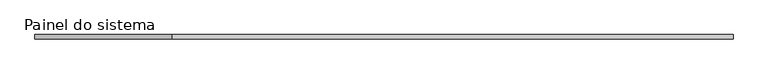
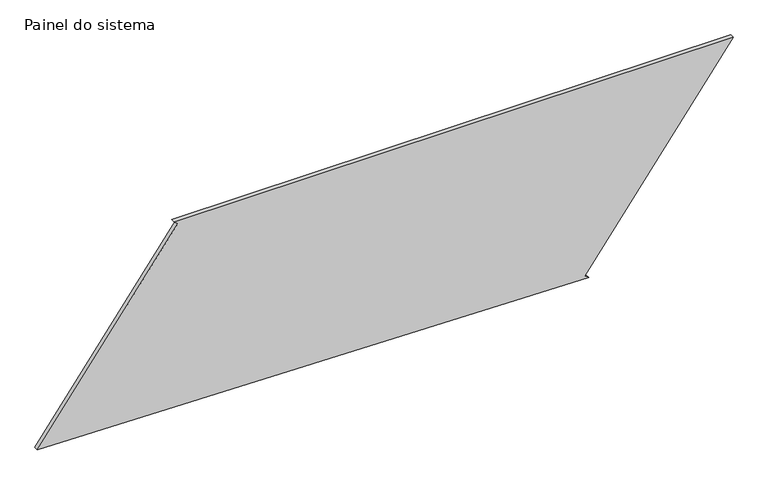
"""IFC4 building model written with IfcOpenShell, lengths in millimetres: plate geometry, Painel do sistema : Envidraçado."""

from ifc_helpers import new_model, si_unit, frame, origin, place, context, project, spatial, polyline, outline, extrude, source, transform, mapped, element, save


def painel_do_sistema_4a3dac21(model_context):
    return source(origin(), model_context, "Body", "SweptSolid", [
        extrude(outline(polyline([(0.0, 1151.4554334), (14.8374505, 1131.3345471), (1152.4919484, 1970.2584434), (1152.4919484, -1195.1450429), (1137.6544979, -1175.0241566), (59.2469484, -1970.2584434), (0.0, 1151.4554334)])), frame((0.0, 24.5, 0.0), z_axis=(0.0, 1.0, 0.0), x_axis=(0.0, 0.0, 1.0)), (0.0, 0.0, 1.0), 25.0),
    ])


if __name__ == "__main__":
    model = new_model("IFC4")
    model_context = context("Model", 3, world=origin())
    ifc_project = project(units=[si_unit("LENGTHUNIT", "METRE", prefix="MILLI")], contexts=[model_context])
    site = spatial("IfcSite", under=ifc_project)
    building = spatial("IfcBuilding", under=site)
    placement = place(None, origin())
    painel_do_sistema_shape = painel_do_sistema_4a3dac21(model_context)
    element("IfcPlate", 1, ObjectType="Painel do sistema : Envidraçado", at=placement, inside=building, context=model_context, shape_type="MappedRepresentation", body=[
        mapped(painel_do_sistema_shape, transform((0.0, 0.0, 0.0), x_axis=(1.0, 0.0, 0.0), y_axis=(0.0, 1.0, 0.0), z_axis=(0.0, 0.0, 1.0))),
    ])
    save(model, "model.ifc")

# Revit data of these elements
# Type "Painel do sistema : Envidraçado"
#   Construction Type Id = "GSP4R"
#   Analytic Construction = "Vidraça única Pilkington 1/8 pol"
#   Visual Light Transmittance = 0.9
#   Solar Heat Gain Coefficient = 0.86
#   Heat Transfer Coefficient (U) = 6.7069 W/(m²·K)
# Element 1 (IfcPlate, "Painel do sistema : Envidraçado")
#   Materials on its faces: "Vidro"
# Materials
#   "Vidro": class "Vidro", colour RGB 0 128 192, transparency 0.9, Description = "Vidro de sílica", Cost = 0
